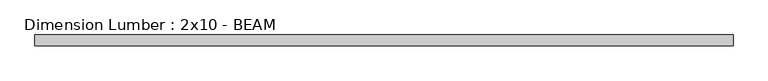
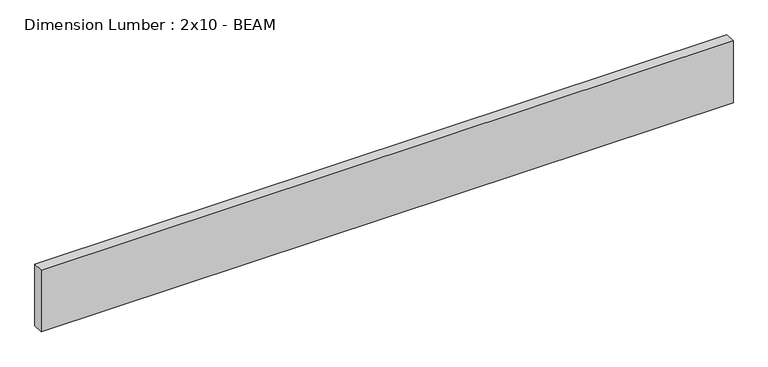
"""IFC4 building model written with IfcOpenShell, lengths in millimetres: beam geometry, Dimension Lumber : 2x10 - BEAM."""

from ifc_helpers import new_model, si_unit, frame, origin, place, context, project, spatial, polyline, outline, extrude, source, transform, mapped, element, save


def dimension_lumber_2x10_beam_43e97269(model_context):
    return source(origin(), model_context, "Body", "SweptSolid", [
        extrude(outline(polyline([(1191.2663185, 19.05), (1191.2663185, -19.05), (-1300.8038185, -19.05), (-1300.8038185, 19.05), (1191.2663185, 19.05)])), frame((0.0, 0.0, -117.475), z_axis=(0.0, 0.0, 1.0), x_axis=(1.0, 0.0, 0.0)), (0.0, 0.0, 1.0), 234.95),
    ])


if __name__ == "__main__":
    model = new_model("IFC4")
    model_context = context("Model", 3, world=origin())
    ifc_project = project(units=[si_unit("LENGTHUNIT", "METRE", prefix="MILLI")], contexts=[model_context])
    site = spatial("IfcSite", under=ifc_project)
    building = spatial("IfcBuilding", under=site)
    placement = place(None, origin())
    dimension_lumber_2x10_beam_shape = dimension_lumber_2x10_beam_43e97269(model_context)
    element("IfcBeam", 1, ObjectType="Dimension Lumber : 2x10 - BEAM", at=placement, inside=building, context=model_context, shape_type="MappedRepresentation", body=[
        mapped(dimension_lumber_2x10_beam_shape, transform((0.0, 0.0, 0.0), x_axis=(1.0, 0.0, 0.0), y_axis=(0.0, 1.0, 0.0), z_axis=(0.0, 0.0, 1.0))),
    ])
    save(model, "model.ifc")

# Revit data of these elements
# Type "Dimension Lumber : 2x10 - BEAM"
#   Assembly Code = "B10"
#   A = 0.0755556 SF
#   Length [instance default] = 5' - 0"
#   b = 0' - 1 1/2"
#   d = 0' - 9 1/4"
#   Structural Material = (3) SISTERED 2X10s AT BEAM
# Element 1 (IfcBeam, "Dimension Lumber : 2x10 - BEAM")
#   Materials on its faces: "(3) SISTERED 2X10s AT BEAM"
# Materials
#   "(3) SISTERED 2X10s AT BEAM": class "Wood", colour RGB 234 198 147, transparency 0, Description = "Pinus Echinata", Cost = 0
